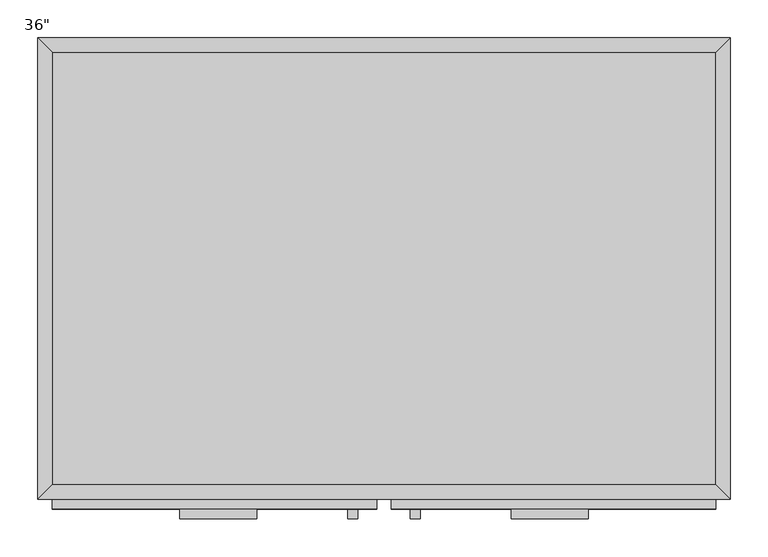
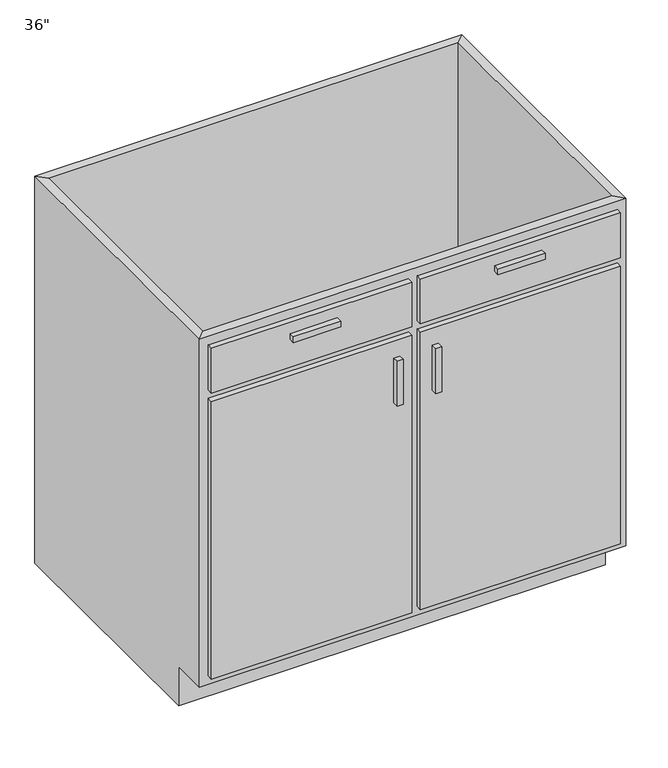
"""IFC4 building model written with IfcOpenShell, lengths in millimetres: furniture geometry."""

from ifc_helpers import new_model, si_unit, frame, origin, place, context, project, spatial, polyline, outline, extrude, faceted_brep, source, transform, mapped, element, save


def furniture_b6fbc004(model_context):
    return source(origin(), model_context, "Body", "SolidModel", [
        faceted_brep([(456.8877049, -590.55, 876.3), (456.8877049, -590.55, 88.9), (-419.4122951, -590.55, 88.9), (-419.4122951, -590.55, 876.3), (-438.4622951, -609.6, 876.3), (475.9377049, -609.6, 876.3), (-438.4622951, -609.6, 88.9), (475.9377049, -609.6, 88.9), (-419.4122951, -533.4, 88.9), (-419.4122951, -19.05, 88.9), (-419.4122951, -19.05, 876.3), (-438.4622951, 0.0, 876.3), (-438.4622951, 0.0, 0.0), (-438.4622951, -533.4, 0.0), (-438.4622951, -533.4, 88.9), (456.8877049, -19.05, 88.9), (456.8877049, -19.05, 876.3), (475.9377049, 0.0, 876.3), (475.9377049, 0.0, 0.0), (456.8877049, -533.4, 88.9), (475.9377049, -533.4, 88.9), (475.9377049, -533.4, 0.0)], [[[0, 1, 2, 3]], [[0, 3, 4, 5]], [[5, 4, 6, 7]], [[2, 1, 7, 6]], [[3, 2, 8, 9, 10]], [[4, 3, 10, 11]], [[6, 4, 11, 12, 13, 14]], [[2, 6, 14, 8]], [[10, 9, 15, 16]], [[11, 10, 16, 17]], [[12, 11, 17, 18]], [[1, 0, 16, 15, 19]], [[0, 5, 17, 16]], [[5, 7, 20, 21, 18, 17]], [[7, 1, 19, 20]], [[8, 19, 15, 9]], [[18, 21, 13, 12]], [[13, 21, 20, 19, 8, 14]]]),
        extrude(outline(polyline([(-149.5372951, -635.0), (-251.1372951, -635.0), (-251.1372951, -622.3), (-149.5372951, -622.3), (-149.5372951, -635.0)])), frame((0.0, 0.0, 819.15), z_axis=(0.0, 0.0, 1.0), x_axis=(1.0, 0.0, 0.0)), (0.0, 0.0, 1.0), 12.7),
        extrude(outline(polyline([(288.6127049, -635.0), (187.0127049, -635.0), (187.0127049, -622.3), (288.6127049, -622.3), (288.6127049, -635.0)])), frame((0.0, 0.0, 819.15), z_axis=(0.0, 0.0, 1.0), x_axis=(1.0, 0.0, 0.0)), (0.0, 0.0, 1.0), 12.7),
        extrude(outline(polyline([(-16.1872951, -635.0), (-28.8872951, -635.0), (-28.8872951, -622.3), (-16.1872951, -622.3), (-16.1872951, -635.0)])), frame((0.0, 0.0, 596.9), z_axis=(0.0, 0.0, 1.0), x_axis=(1.0, 0.0, 0.0)), (0.0, 0.0, 1.0), 101.6),
        extrude(outline(polyline([(66.3627049, -635.0), (53.6627049, -635.0), (53.6627049, -622.3), (66.3627049, -622.3), (66.3627049, -635.0)])), frame((0.0, 0.0, 596.9), z_axis=(0.0, 0.0, 1.0), x_axis=(1.0, 0.0, 0.0)), (0.0, 0.0, 1.0), 101.6),
        extrude(outline(polyline([(456.8877049, -19.05), (456.8877049, -590.55), (-419.4122951, -590.55), (-419.4122951, -19.05), (456.8877049, -19.05)])), frame((0.0, 0.0, 88.9), z_axis=(0.0, 0.0, 1.0), x_axis=(1.0, 0.0, 0.0)), (0.0, 0.0, 1.0), 19.05),
        extrude(outline(polyline([(9.2127049, -622.3), (-419.4122951, -622.3), (-419.4122951, -609.6), (9.2127049, -609.6), (9.2127049, -622.3)])), frame((0.0, 0.0, 755.65), z_axis=(0.0, 0.0, 1.0), x_axis=(1.0, 0.0, 0.0)), (0.0, 0.0, 1.0), 101.6),
        extrude(outline(polyline([(456.8877049, -622.3), (28.2627049, -622.3), (28.2627049, -609.6), (456.8877049, -609.6), (456.8877049, -622.3)])), frame((0.0, 0.0, 755.65), z_axis=(0.0, 0.0, 1.0), x_axis=(1.0, 0.0, 0.0)), (0.0, 0.0, 1.0), 101.6),
        extrude(outline(polyline([(9.2127049, -622.3), (-419.4122951, -622.3), (-419.4122951, -609.6), (9.2127049, -609.6), (9.2127049, -622.3)])), frame((0.0, 0.0, 107.95), z_axis=(0.0, 0.0, 1.0), x_axis=(1.0, 0.0, 0.0)), (0.0, 0.0, 1.0), 628.65),
        extrude(outline(polyline([(456.8877049, -622.3), (28.2627049, -622.3), (28.2627049, -609.6), (456.8877049, -609.6), (456.8877049, -622.3)])), frame((0.0, 0.0, 107.95), z_axis=(0.0, 0.0, 1.0), x_axis=(1.0, 0.0, 0.0)), (0.0, 0.0, 1.0), 628.65),
    ])


if __name__ == "__main__":
    model = new_model("IFC4")
    model_context = context("Model", 3, world=origin())
    ifc_project = project(units=[si_unit("LENGTHUNIT", "METRE", prefix="MILLI")], contexts=[model_context])
    site = spatial("IfcSite", under=ifc_project)
    building = spatial("IfcBuilding", under=site)
    placement = place(None, origin())
    furniture_shape = furniture_b6fbc004(model_context)
    element("IfcFurniture", 1, ObjectType="Base Cabinet-Double Door & 2 Drawer : 36\"", at=placement, inside=building, context=model_context, shape_type="MappedRepresentation", body=[
        mapped(furniture_shape, transform((0.0, 0.0, 0.0), x_axis=(1.0, 0.0, 0.0), y_axis=(0.0, 1.0, 0.0), z_axis=(0.0, 0.0, 1.0))),
    ])
    save(model, "model.ifc")

# Revit data of these elements
# Type "Base Cabinet-Double Door & 2 Drawer : 36\""
#   Assembly Code = "C1030410"
#   Depth = 2' - 0"
#   Height = 2' - 10 1/2"
#   Toe Depth = 0' - 3"
#   Toe Height = 0' - 3 1/2"
#   Width = 3' - 0"
#   Cabinet Material = none
#   Door/Drawer Material = none
#   Handle Material = Cabinets - Handles
#   Default Elevation = 0
# Element 1 (IfcFurniture, "Base Cabinet-Double Door & 2 Drawer : 36\"")
#   Materials on its faces: "Cabinets", "Cabinets - Handles"
# Materials
#   "Cabinets - Handles": class "Metal", colour RGB 57 57 57, transparency 0
#   "Cabinets": class "Miscellaneous", colour RGB 249 249 249, transparency 0
